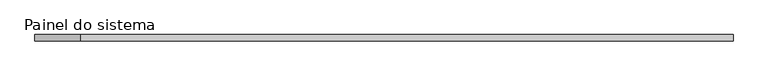
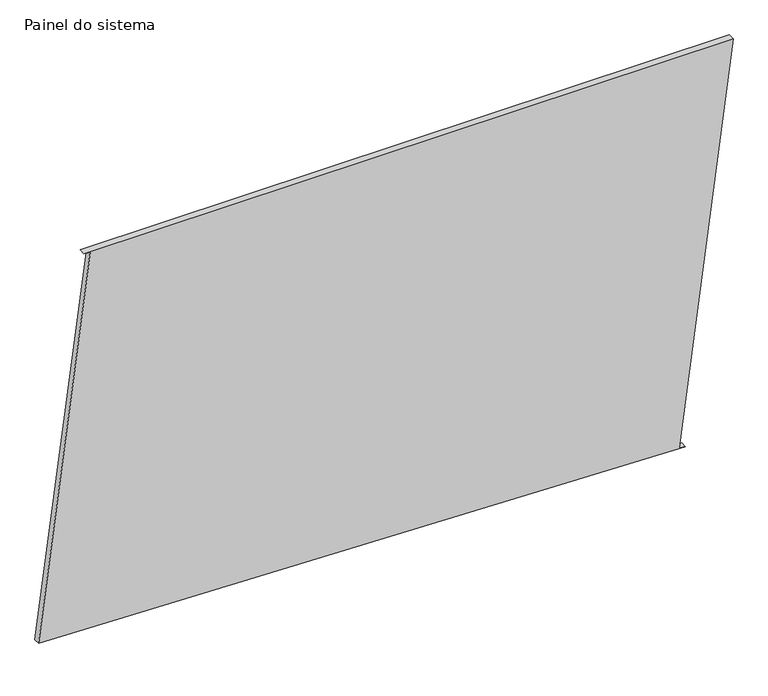
"""IFC4 building model written with IfcOpenShell, lengths in millimetres: plate geometry, Painel do sistema : Envidraçado."""

from ifc_helpers import new_model, si_unit, frame, origin, place, context, project, spatial, polyline, outline, extrude, source, transform, mapped, element, save


def painel_do_sistema_e402e947(model_context):
    return source(origin(), model_context, "Body", "SweptSolid", [
        extrude(outline(polyline([(0.0, 1185.298359), (3.2380023, 1160.508939), (1641.0279418, 1374.4376048), (1641.0279418, -1194.8328174), (1637.7899395, -1170.0433974), (72.9936776, -1374.4376048), (0.0, 1185.298359)])), frame((0.0, 24.5, 0.0), z_axis=(0.0, 1.0, 0.0), x_axis=(0.0, 0.0, 1.0)), (0.0, 0.0, 1.0), 25.0),
    ])


if __name__ == "__main__":
    model = new_model("IFC4")
    model_context = context("Model", 3, world=origin())
    ifc_project = project(units=[si_unit("LENGTHUNIT", "METRE", prefix="MILLI")], contexts=[model_context])
    site = spatial("IfcSite", under=ifc_project)
    building = spatial("IfcBuilding", under=site)
    placement = place(None, origin())
    painel_do_sistema_shape = painel_do_sistema_e402e947(model_context)
    element("IfcPlate", 1, ObjectType="Painel do sistema : Envidraçado", at=placement, inside=building, context=model_context, shape_type="MappedRepresentation", body=[
        mapped(painel_do_sistema_shape, transform((0.0, 0.0, 0.0), x_axis=(1.0, 0.0, 0.0), y_axis=(0.0, 1.0, 0.0), z_axis=(0.0, 0.0, 1.0))),
    ])
    save(model, "model.ifc")

# Revit data of these elements
# Type "Painel do sistema : Envidraçado"
#   Construction Type Id = "GSP4R"
#   Analytic Construction = "Vidraça única Pilkington 1/8 pol"
#   Visual Light Transmittance = 0.9
#   Solar Heat Gain Coefficient = 0.86
#   Heat Transfer Coefficient (U) = 6.7069 W/(m²·K)
# Element 1 (IfcPlate, "Painel do sistema : Envidraçado")
#   Materials on its faces: "Vidro"
# Materials
#   "Vidro": class "Vidro", colour RGB 0 128 192, transparency 0.9, Description = "Vidro de sílica", Cost = 0
